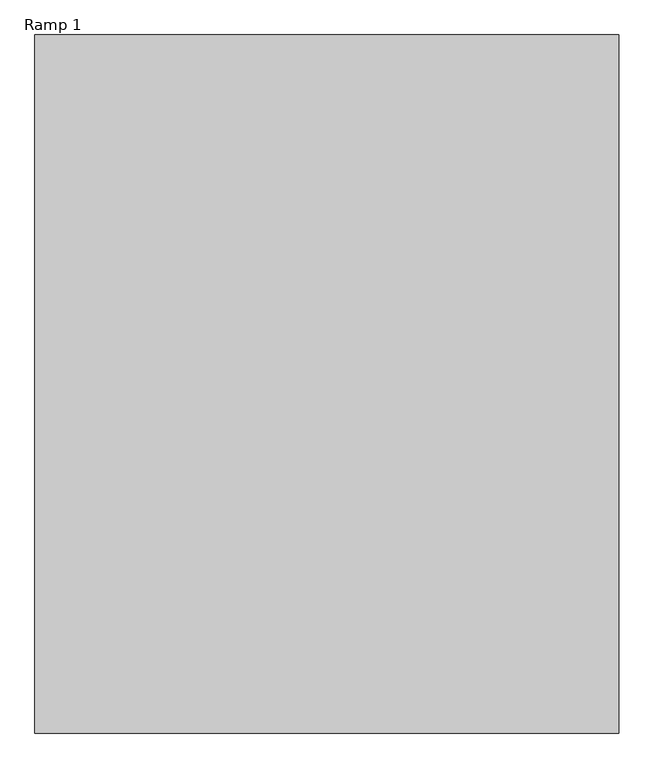
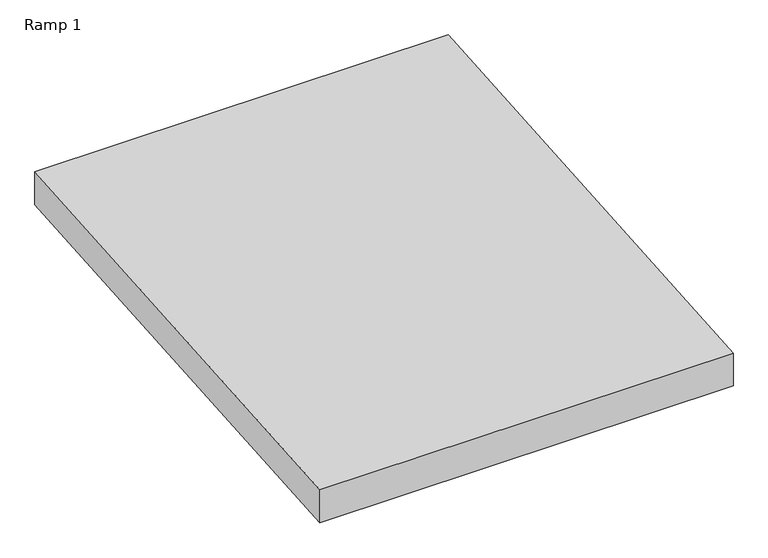
"""IFC4 building model written with IfcOpenShell, lengths in millimetres: ramp geometry, Ramp 1."""

from ifc_helpers import new_model, si_unit, frame, origin, place, context, project, spatial, polyline, outline, extrude, source, transform, mapped, element, save


def ramp_1_445c0b72(model_context):
    return source(origin(), model_context, "Body", "SweptSolid", [
        extrude(outline(polyline([(-378.9025016, 40.0), (1760.7723822, 200.0), (1760.7723822, 49.5812066), (-378.9025016, -110.4187934), (-378.9025016, 40.0)])), frame((5764.7203549, 0.0, 0.0), z_axis=(1.0, 0.0, 0.0), x_axis=(0.0, 1.0, 0.0)), (0.0, 0.0, 1.0), 1790.0),
    ])


if __name__ == "__main__":
    model = new_model("IFC4")
    model_context = context("Model", 3, world=origin())
    ifc_project = project(units=[si_unit("LENGTHUNIT", "METRE", prefix="MILLI")], contexts=[model_context])
    site = spatial("IfcSite", under=ifc_project)
    building = spatial("IfcBuilding", under=site)
    placement = place(None, origin())
    ramp_1_shape = ramp_1_445c0b72(model_context)
    element("IfcRamp", 1, ObjectType="Ramp 1", at=placement, inside=building, context=model_context, shape_type="MappedRepresentation", body=[
        mapped(ramp_1_shape, transform((0.0, 0.0, 0.0), x_axis=(1.0, 0.0, 0.0), y_axis=(0.0, 1.0, 0.0), z_axis=(0.0, 0.0, 1.0))),
    ])
    save(model, "model.ifc")
